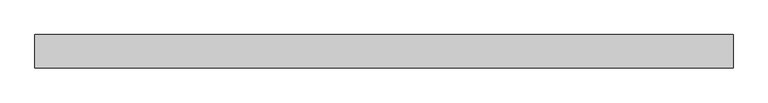
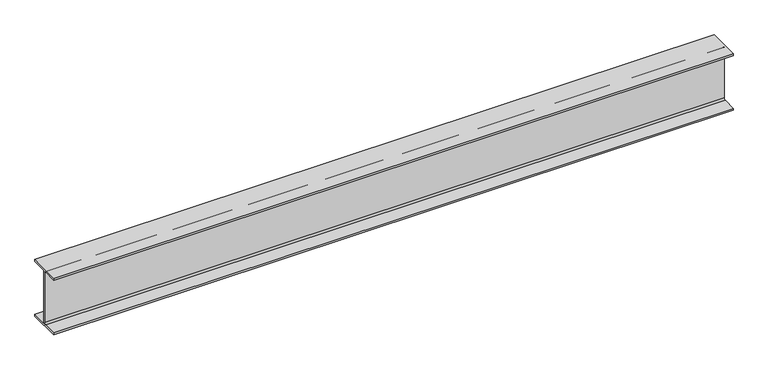
"""IFC4 building model written with IfcOpenShell, lengths in millimetres: beam geometry, Steel Beam_H-KSD3502 : H_SB_ASB_H-200x200x8x12."""

from ifc_helpers import new_model, si_unit, point, frame, frame_2d, origin, place, context, project, spatial, polyline, circle_curve, trimmed, segment, composite_curve, outline, extrude, source, transform, mapped, element, save


def beam_9a6c1f0b(model_context):
    return source(origin(), model_context, "Body", "SweptSolid", [
        extrude(outline(composite_curve([segment(polyline([(82.5, -141.5), (82.5, -151.7), (-82.5, -151.7), (-82.5, -141.5), (-11.9, -141.5)]), True, "CONTINUOUS"), segment(trimmed(circle_curve(frame_2d((-11.9, -132.6)), 8.9), [point((-11.9, -141.5))], [point((-3.0, -132.6))], True, "CARTESIAN"), True, "CONTINUOUS"), segment(polyline([(-3.0, -132.6), (-3.0, 132.6)]), True, "CONTINUOUS"), segment(trimmed(circle_curve(frame_2d((-11.9, 132.6)), 8.9), [point((-3.0, 132.6))], [point((-11.9, 141.5))], True, "CARTESIAN"), True, "CONTINUOUS"), segment(polyline([(-11.9, 141.5), (-82.5, 141.5), (-82.5, 151.7), (82.5, 151.7), (82.5, 141.5), (11.9, 141.5)]), True, "CONTINUOUS"), segment(trimmed(circle_curve(frame_2d((11.9, 132.6)), 8.9), [point((11.9, 141.5))], [point((3.0, 132.6))], True, "CARTESIAN"), True, "CONTINUOUS"), segment(polyline([(3.0, 132.6), (3.0, -132.6)]), True, "CONTINUOUS"), segment(trimmed(circle_curve(frame_2d((11.9, -132.6)), 8.9), [point((3.0, -132.6))], [point((11.9, -141.5))], True, "CARTESIAN"), True, "CONTINUOUS"), segment(polyline([(11.9, -141.5), (82.5, -141.5)]), True, "CONTINUOUS")], self_intersect=False)), frame((-1601.8217098, 0.0, 0.0), z_axis=(1.0, 0.0, 0.0), x_axis=(0.0, 1.0, 0.0)), (0.0, 0.0, 1.0), 3433.6669039),
    ])


if __name__ == "__main__":
    model = new_model("IFC4")
    model_context = context("Model", 3, world=origin())
    ifc_project = project(units=[si_unit("LENGTHUNIT", "METRE", prefix="MILLI")], contexts=[model_context])
    site = spatial("IfcSite", under=ifc_project)
    building = spatial("IfcBuilding", under=site)
    placement = place(None, origin())
    beam_shape = beam_9a6c1f0b(model_context)
    element("IfcBeam", 1, ObjectType="Steel Beam_H-KSD3502 : H_SB_ASB_H-200x200x8x12", at=placement, inside=building, context=model_context, shape_type="MappedRepresentation", body=[
        mapped(beam_shape, transform((0.0, 0.0, 0.0), x_axis=(1.0, 0.0, 0.0), y_axis=(0.0, 1.0, 0.0), z_axis=(0.0, 0.0, 1.0))),
    ])
    save(model, "model.ifc")

# Revit data of these elements
# Type "Steel Beam_H-KSD3502 : H_SB_ASB_H-200x200x8x12"
#   Width = 20.0 cm
#   Web Thickness = 0.8 cm
#   Web Fillet = 1.3 cm
#   Warping Constant = 141376.0 cm⁶
#   Torsional Moment of Inertia = 26.2485 cm⁴
#   Torsional Modulus = 1.0 cm³
#   Section Area = 63.53 cm²
#   Plastic Modulus weak axis = 244.0 cm³
#   Plastic Modulus strong axis = 525.0 cm³
#   Perimeter = 1.16 m²/m
#   Nominal Weight = 49.90 kgf/m
#   Moment of Inertia weak axis = 1600.00 cm⁴
#   Moment of Inertia strong axis = 4720.00 cm⁴
#   Height = 20.0 cm
#   Flange Thickness = 1.2 cm
#   Elastic Modulus weak axis = 160.0 cm³
#   Elastic Modulus strong axis = 472.0 cm³
#   Centroid Vertical = 10.0 cm
#   Centroid Horizontal = 10.0 cm
#   Length [instance default] = 1.5240 m
#   Structural Material [instance default] = Steel, 45-345
#   Assembly Code = ""
# Element 1 (IfcBeam, "Steel Beam_H-KSD3502 : H_SB_ASB_H-200x200x8x12")
#   Structural Material = none
# Materials
#   "Steel, 45-345": class "Metal", colour RGB 189 187 185, transparency 0, Description = "Steel 345 MPa", Cost = 0
